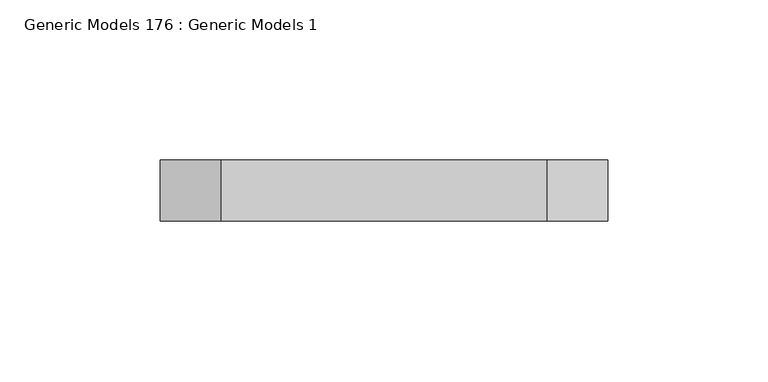
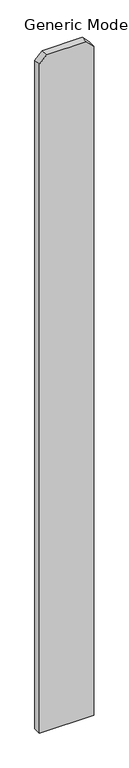
"""IFC4 building model written with IfcOpenShell, lengths in millimetres: proxy geometry, Generic Models 176 : Generic Models 1."""

from ifc_helpers import new_model, si_unit, frame, origin, place, context, project, spatial, polyline, outline, extrude, source, transform, mapped, element, save


def generic_models_176_generic_models_1_de16f722(model_context):
    return source(origin(), model_context, "Body", "SweptSolid", [
        extrude(outline(polyline([(76.2, 56818.2125), (1885.95, 56818.2125), (1905.0, 56799.1625), (1905.0, 56697.5625), (1885.95, 56678.5125), (76.2, 56678.5125), (76.2, 56818.2125)])), frame((0.0, 547.6875, 0.0), z_axis=(0.0, 1.0, 0.0), x_axis=(0.0, 0.0, 1.0)), (0.0, 0.0, 1.0), 19.05),
    ])


if __name__ == "__main__":
    model = new_model("IFC4")
    model_context = context("Model", 3, world=origin())
    ifc_project = project(units=[si_unit("LENGTHUNIT", "METRE", prefix="MILLI")], contexts=[model_context])
    site = spatial("IfcSite", under=ifc_project)
    building = spatial("IfcBuilding", under=site)
    placement = place(None, origin())
    generic_models_176_generic_models_1_shape = generic_models_176_generic_models_1_de16f722(model_context)
    element("IfcBuildingElementProxy", 1, Name="Generic Models 176 : Generic Models 1", ObjectType="Generic Models 176 : Generic Models 1", at=placement, inside=building, context=model_context, shape_type="MappedRepresentation", body=[
        mapped(generic_models_176_generic_models_1_shape, transform((0.0, 0.0, 0.0), x_axis=(1.0, 0.0, 0.0), y_axis=(0.0, 1.0, 0.0), z_axis=(0.0, 0.0, 1.0))),
    ])
    save(model, "model.ifc")

# Revit data of these elements
# Element 1 (IfcBuildingElementProxy, "Generic Models 176 : Generic Models 1")
#   Materials on its faces: "VERTICAL 1X6 CEDAR PLANKS W/ CLEAR WOOD SEALER"
# Materials
#   "VERTICAL 1X6 CEDAR PLANKS W/ CLEAR WOOD SEALER": class "Wood", colour RGB 234 198 147, transparency 0, Description = "Pinus Echinata", Cost = 0
